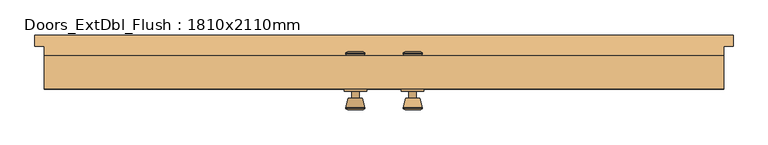
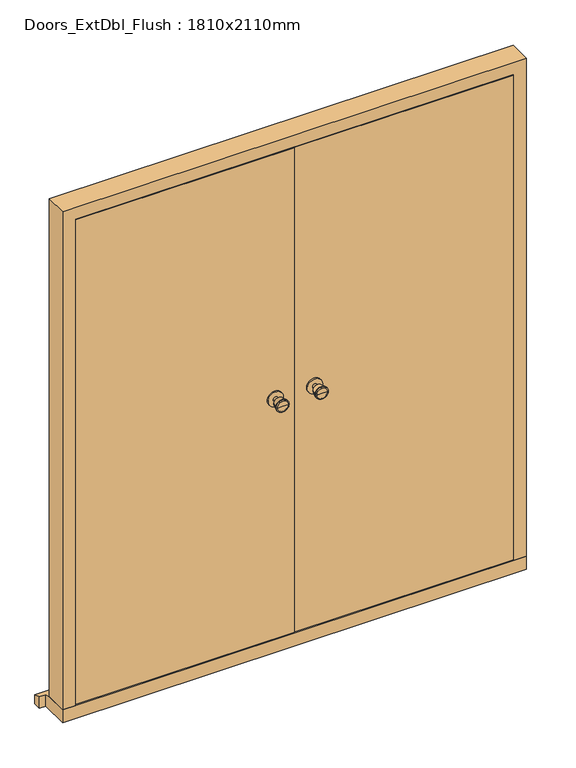
"""IFC4 building model written with IfcOpenShell, lengths in millimetres: door geometry, Doors_ExtDbl_Flush : 1810x2110mm."""

from ifc_helpers import new_model, si_unit, point, frame, frame_2d, origin, place, context, project, spatial, polyline, circle_curve, trimmed, segment, composite_curve, outline, extrude, faceted_brep, source, transform, mapped, element, save
from ifc_brep_helpers import plane_surface, cylinder_surface, revolved_surface, advanced_brep


def doors_extdbl_flush_1810x2110mm_ef948ade(model_context):
    return source(origin(), model_context, "Body", "SolidModel", [
        advanced_brep(
        [(-76.5, -57.5, 1050.0), (-66.5, -57.5, 1050.0), (-86.5, -57.5, 1050.0), (-96.9758676, -106.5, 1050.0), (-56.0241324, -106.5, 1050.0), (-76.5, -106.5, 1050.0), (-101.5, -104.6721319, 1050.0), (-51.5, -104.6721319, 1050.0), (-101.5, -101.2084537, 1050.0), (-51.5, -101.2084537, 1050.0), (-95.136236, -76.5, 1050.0), (-57.863764, -76.5, 1050.0), (-86.5, -76.5, 1050.0), (-66.5, -76.5, 1050.0)],
        [
            (0, 1),
            (1, 2, circle_curve(frame((-76.5, -57.5, 1050.0), z_axis=(0.0, 1.0, 0.0), x_axis=(1.0, 0.0, 0.0)), 10.0)),
            (2, 0),
            (2, 1, circle_curve(frame((-76.5, -57.5, 1050.0), z_axis=(0.0, 1.0, 0.0), x_axis=(1.0, 0.0, 0.0)), 10.0)),
            (3, 4, circle_curve(frame((-76.5, -106.5, 1050.0), z_axis=(0.0, -1.0, 0.0), x_axis=(1.0, 0.0, 0.0)), 20.4758676)),
            (4, 5),
            (5, 3),
            (4, 3, circle_curve(frame((-76.5, -106.5, 1050.0), z_axis=(0.0, -1.0, 0.0), x_axis=(1.0, 0.0, 0.0)), 20.4758676)),
            (6, 7, circle_curve(frame((-76.5, -104.6721319, 1050.0), z_axis=(0.0, -1.0, 0.0), x_axis=(1.0, 0.0, 0.0)), 25.0)),
            (7, 4),
            (3, 6),
            (7, 6, circle_curve(frame((-76.5, -104.6721319, 1050.0), z_axis=(0.0, -1.0, 0.0), x_axis=(1.0, 0.0, 0.0)), 25.0)),
            (8, 9, circle_curve(frame((-76.5, -101.2084537, 1050.0), z_axis=(0.0, -1.0, 0.0), x_axis=(1.0, 0.0, 0.0)), 25.0)),
            (9, 7),
            (6, 8),
            (9, 8, circle_curve(frame((-76.5, -101.2084537, 1050.0), z_axis=(0.0, -1.0, 0.0), x_axis=(1.0, 0.0, 0.0)), 25.0)),
            (10, 11, circle_curve(frame((-76.5, -76.5, 1050.0), z_axis=(0.0, -1.0, 0.0), x_axis=(1.0, 0.0, 0.0)), 18.636236)),
            (11, 9),
            (8, 10),
            (11, 10, circle_curve(frame((-76.5, -76.5, 1050.0), z_axis=(0.0, -1.0, 0.0), x_axis=(1.0, 0.0, 0.0)), 18.636236)),
            (12, 13, circle_curve(frame((-76.5, -76.5, 1050.0), z_axis=(0.0, -1.0, 0.0), x_axis=(1.0, 0.0, 0.0)), 10.0)),
            (13, 11),
            (10, 12),
            (13, 12, circle_curve(frame((-76.5, -76.5, 1050.0), z_axis=(0.0, -1.0, 0.0), x_axis=(1.0, 0.0, 0.0)), 10.0)),
            (1, 13),
            (12, 2),
        ],
        [
            plane_surface(frame((-76.5, -57.5, 1050.0), z_axis=(0.0, 1.0, 0.0), x_axis=(1.0, 0.0, 0.0))),
            plane_surface(frame((-76.5, -106.5, 1050.0), z_axis=(0.0, -1.0, 0.0), x_axis=(1.0, 0.0, 0.0))),
            revolved_surface(polyline([(-56.0241324, -106.5, 1050.0), (-51.5, -104.6721319, 1050.0)]), (-76.5, -57.5, 1050.0), (0.0, 1.0, 0.0)),
            cylinder_surface(frame((-76.5, -57.5, 1050.0), z_axis=(0.0, 1.0, 0.0), x_axis=(1.0, 0.0, 0.0)), 25.0),
            revolved_surface(polyline([(-51.5, -101.2084537, 1050.0), (-57.863764, -76.5, 1050.0)]), (-76.5, -57.5, 1050.0), (0.0, 1.0, 0.0)),
            plane_surface(frame((-76.5, -76.5, 1050.0), z_axis=(0.0, 1.0, 0.0), x_axis=(1.0, 0.0, 0.0))),
            cylinder_surface(frame((-76.5, -57.5, 1050.0), z_axis=(0.0, 1.0, 0.0), x_axis=(1.0, 0.0, 0.0)), 10.0),
        ],
        [
            (0, [[1, 2, 3]]),
            (0, [[-3, 4, -1]]),
            (1, [[5, 6, 7]]),
            (1, [[8, -7, -6]]),
            (2, [[9, 10, -5, 11]]),
            (2, [[12, -11, -8, -10]]),
            (3, [[13, 14, -9, 15]]),
            (3, [[16, -15, -12, -14]]),
            (4, [[17, 18, -13, 19]]),
            (4, [[20, -19, -16, -18]]),
            (5, [[21, 22, -17, 23]]),
            (5, [[24, -23, -20, -22]]),
            (6, [[-2, 25, -21, 26]]),
            (6, [[-4, -26, -24, -25]]),
        ],
    ),
        extrude(outline(composite_curve([segment(trimmed(circle_curve(frame_2d((1050.0, -76.5)), 30.0), [point((1050.0, -46.5))], [point((1050.0, -106.5))], False, "CARTESIAN"), True, "CONTINUOUS"), segment(trimmed(circle_curve(frame_2d((1050.0, -76.5)), 30.0), [point((1050.0, -106.5))], [point((1050.0, -46.5))], False, "CARTESIAN"), True, "CONTINUOUS")], self_intersect=False)), frame((0.0, -57.5, 0.0), z_axis=(0.0, 1.0, 0.0), x_axis=(0.0, 0.0, 1.0)), (0.0, 0.0, 1.0), 6.0),
        advanced_brep(
        [(-76.5, -1.5, 1050.0), (-86.5, -1.5, 1050.0), (-66.5, -1.5, 1050.0), (-96.9758676, 47.5, 1050.0), (-76.5, 47.5, 1050.0), (-56.0241324, 47.5, 1050.0), (-101.5, 45.6721319, 1050.0), (-51.5, 45.6721319, 1050.0), (-101.5, 42.2084537, 1050.0), (-51.5, 42.2084537, 1050.0), (-95.136236, 17.5, 1050.0), (-57.863764, 17.5, 1050.0), (-86.5, 17.5, 1050.0), (-66.5, 17.5, 1050.0)],
        [
            (0, 1),
            (1, 2, circle_curve(frame((-76.5, -1.5, 1050.0), z_axis=(0.0, -1.0, 0.0), x_axis=(1.0, 0.0, 0.0)), 10.0)),
            (2, 0),
            (2, 1, circle_curve(frame((-76.5, -1.5, 1050.0), z_axis=(0.0, -1.0, 0.0), x_axis=(1.0, 0.0, 0.0)), 10.0)),
            (3, 4),
            (4, 5),
            (5, 3, circle_curve(frame((-76.5, 47.5, 1050.0), z_axis=(0.0, 1.0, 0.0), x_axis=(1.0, 0.0, 0.0)), 20.4758676)),
            (3, 5, circle_curve(frame((-76.5, 47.5, 1050.0), z_axis=(0.0, 1.0, 0.0), x_axis=(1.0, 0.0, 0.0)), 20.4758676)),
            (6, 3),
            (5, 7),
            (7, 6, circle_curve(frame((-76.5, 45.6721319, 1050.0), z_axis=(0.0, 1.0, 0.0), x_axis=(1.0, 0.0, 0.0)), 25.0)),
            (6, 7, circle_curve(frame((-76.5, 45.6721319, 1050.0), z_axis=(0.0, 1.0, 0.0), x_axis=(1.0, 0.0, 0.0)), 25.0)),
            (8, 6),
            (7, 9),
            (9, 8, circle_curve(frame((-76.5, 42.2084537, 1050.0), z_axis=(0.0, 1.0, 0.0), x_axis=(1.0, 0.0, 0.0)), 25.0)),
            (8, 9, circle_curve(frame((-76.5, 42.2084537, 1050.0), z_axis=(0.0, 1.0, 0.0), x_axis=(1.0, 0.0, 0.0)), 25.0)),
            (10, 8),
            (9, 11),
            (11, 10, circle_curve(frame((-76.5, 17.5, 1050.0), z_axis=(0.0, 1.0, 0.0), x_axis=(1.0, 0.0, 0.0)), 18.636236)),
            (10, 11, circle_curve(frame((-76.5, 17.5, 1050.0), z_axis=(0.0, 1.0, 0.0), x_axis=(1.0, 0.0, 0.0)), 18.636236)),
            (12, 10),
            (11, 13),
            (13, 12, circle_curve(frame((-76.5, 17.5, 1050.0), z_axis=(0.0, 1.0, 0.0), x_axis=(1.0, 0.0, 0.0)), 10.0)),
            (12, 13, circle_curve(frame((-76.5, 17.5, 1050.0), z_axis=(0.0, 1.0, 0.0), x_axis=(1.0, 0.0, 0.0)), 10.0)),
            (1, 12),
            (13, 2),
        ],
        [
            plane_surface(frame((-76.5, -1.5, 1050.0), z_axis=(0.0, -1.0, 0.0), x_axis=(1.0, 0.0, 0.0))),
            plane_surface(frame((-76.5, 47.5, 1050.0), z_axis=(0.0, 1.0, 0.0), x_axis=(1.0, 0.0, 0.0))),
            revolved_surface(polyline([(-56.0241324, 47.5, 1050.0), (-51.5, 45.6721319, 1050.0)]), (-76.5, -1.5, 1050.0), (0.0, -1.0, 0.0)),
            cylinder_surface(frame((-76.5, -1.5, 1050.0), z_axis=(0.0, -1.0, 0.0), x_axis=(1.0, 0.0, 0.0)), 25.0),
            revolved_surface(polyline([(-51.5, 42.2084537, 1050.0), (-57.863764, 17.5, 1050.0)]), (-76.5, -1.5, 1050.0), (0.0, -1.0, 0.0)),
            plane_surface(frame((-76.5, 17.5, 1050.0), z_axis=(0.0, -1.0, 0.0), x_axis=(1.0, 0.0, 0.0))),
            cylinder_surface(frame((-76.5, -1.5, 1050.0), z_axis=(0.0, -1.0, 0.0), x_axis=(1.0, 0.0, 0.0)), 10.0),
        ],
        [
            (0, [[1, 2, 3]]),
            (0, [[-3, 4, -1]]),
            (1, [[5, 6, 7]]),
            (1, [[-6, -5, 8]]),
            (2, [[9, -7, 10, 11]]),
            (2, [[-10, -8, -9, 12]]),
            (3, [[13, -11, 14, 15]]),
            (3, [[-14, -12, -13, 16]]),
            (4, [[17, -15, 18, 19]]),
            (4, [[-18, -16, -17, 20]]),
            (5, [[21, -19, 22, 23]]),
            (5, [[-22, -20, -21, 24]]),
            (6, [[25, -23, 26, -2]]),
            (6, [[-26, -24, -25, -4]]),
        ],
    ),
        extrude(outline(composite_curve([segment(trimmed(circle_curve(frame_2d((1050.0, -76.5)), 30.0), [point((1050.0, -46.5))], [point((1050.0, -106.5))], False, "CARTESIAN"), True, "CONTINUOUS"), segment(trimmed(circle_curve(frame_2d((1050.0, -76.5)), 30.0), [point((1050.0, -106.5))], [point((1050.0, -46.5))], False, "CARTESIAN"), True, "CONTINUOUS")], self_intersect=False)), frame((0.0, -7.5, 0.0), z_axis=(0.0, 1.0, 0.0), x_axis=(0.0, 0.0, 1.0)), (0.0, 0.0, 1.0), 6.0),
        advanced_brep(
        [(76.5, -57.5, 1050.0), (86.5, -57.5, 1050.0), (66.5, -57.5, 1050.0), (96.9758676, -106.5, 1050.0), (76.5, -106.5, 1050.0), (56.0241324, -106.5, 1050.0), (101.5, -104.6721319, 1050.0), (51.5, -104.6721319, 1050.0), (101.5, -101.2084537, 1050.0), (51.5, -101.2084537, 1050.0), (95.136236, -76.5, 1050.0), (57.863764, -76.5, 1050.0), (86.5, -76.5, 1050.0), (66.5, -76.5, 1050.0)],
        [
            (0, 1),
            (1, 2, circle_curve(frame((76.5, -57.5, 1050.0), z_axis=(0.0, 1.0, 0.0), x_axis=(-1.0, 0.0, 0.0)), 10.0)),
            (2, 0),
            (2, 1, circle_curve(frame((76.5, -57.5, 1050.0), z_axis=(0.0, 1.0, 0.0), x_axis=(-1.0, 0.0, 0.0)), 10.0)),
            (3, 4),
            (4, 5),
            (5, 3, circle_curve(frame((76.5, -106.5, 1050.0), z_axis=(0.0, -1.0, 0.0), x_axis=(-1.0, 0.0, 0.0)), 20.4758676)),
            (3, 5, circle_curve(frame((76.5, -106.5, 1050.0), z_axis=(0.0, -1.0, 0.0), x_axis=(-1.0, 0.0, 0.0)), 20.4758676)),
            (6, 3),
            (5, 7),
            (7, 6, circle_curve(frame((76.5, -104.6721319, 1050.0), z_axis=(0.0, -1.0, 0.0), x_axis=(-1.0, 0.0, 0.0)), 25.0)),
            (6, 7, circle_curve(frame((76.5, -104.6721319, 1050.0), z_axis=(0.0, -1.0, 0.0), x_axis=(-1.0, 0.0, 0.0)), 25.0)),
            (8, 6),
            (7, 9),
            (9, 8, circle_curve(frame((76.5, -101.2084537, 1050.0), z_axis=(0.0, -1.0, 0.0), x_axis=(-1.0, 0.0, 0.0)), 25.0)),
            (8, 9, circle_curve(frame((76.5, -101.2084537, 1050.0), z_axis=(0.0, -1.0, 0.0), x_axis=(-1.0, 0.0, 0.0)), 25.0)),
            (10, 8),
            (9, 11),
            (11, 10, circle_curve(frame((76.5, -76.5, 1050.0), z_axis=(0.0, -1.0, 0.0), x_axis=(-1.0, 0.0, 0.0)), 18.636236)),
            (10, 11, circle_curve(frame((76.5, -76.5, 1050.0), z_axis=(0.0, -1.0, 0.0), x_axis=(-1.0, 0.0, 0.0)), 18.636236)),
            (12, 10),
            (11, 13),
            (13, 12, circle_curve(frame((76.5, -76.5, 1050.0), z_axis=(0.0, -1.0, 0.0), x_axis=(-1.0, 0.0, 0.0)), 10.0)),
            (12, 13, circle_curve(frame((76.5, -76.5, 1050.0), z_axis=(0.0, -1.0, 0.0), x_axis=(-1.0, 0.0, 0.0)), 10.0)),
            (1, 12),
            (13, 2),
        ],
        [
            plane_surface(frame((76.5, -57.5, 1050.0), z_axis=(0.0, 1.0, 0.0), x_axis=(-1.0, 0.0, 0.0))),
            plane_surface(frame((76.5, -106.5, 1050.0), z_axis=(0.0, -1.0, 0.0), x_axis=(-1.0, 0.0, 0.0))),
            revolved_surface(polyline([(56.0241324, -106.5, 1050.0), (51.5, -104.6721319, 1050.0)]), (76.5, -57.5, 1050.0), (0.0, 1.0, 0.0)),
            cylinder_surface(frame((76.5, -57.5, 1050.0), z_axis=(0.0, 1.0, 0.0), x_axis=(-1.0, 0.0, 0.0)), 25.0),
            revolved_surface(polyline([(51.5, -101.2084537, 1050.0), (57.863764, -76.5, 1050.0)]), (76.5, -57.5, 1050.0), (0.0, 1.0, 0.0)),
            plane_surface(frame((76.5, -76.5, 1050.0), z_axis=(0.0, 1.0, 0.0), x_axis=(-1.0, 0.0, 0.0))),
            cylinder_surface(frame((76.5, -57.5, 1050.0), z_axis=(0.0, 1.0, 0.0), x_axis=(-1.0, 0.0, 0.0)), 10.0),
        ],
        [
            (0, [[1, 2, 3]]),
            (0, [[-3, 4, -1]]),
            (1, [[5, 6, 7]]),
            (1, [[-6, -5, 8]]),
            (2, [[9, -7, 10, 11]]),
            (2, [[-10, -8, -9, 12]]),
            (3, [[13, -11, 14, 15]]),
            (3, [[-14, -12, -13, 16]]),
            (4, [[17, -15, 18, 19]]),
            (4, [[-18, -16, -17, 20]]),
            (5, [[21, -19, 22, 23]]),
            (5, [[-22, -20, -21, 24]]),
            (6, [[25, -23, 26, -2]]),
            (6, [[-26, -24, -25, -4]]),
        ],
    ),
        extrude(outline(composite_curve([segment(trimmed(circle_curve(frame_2d((1050.0, 76.5)), 30.0), [point((1050.0, 46.5))], [point((1050.0, 106.5))], False, "CARTESIAN"), True, "CONTINUOUS"), segment(trimmed(circle_curve(frame_2d((1050.0, 76.5)), 30.0), [point((1050.0, 106.5))], [point((1050.0, 46.5))], False, "CARTESIAN"), True, "CONTINUOUS")], self_intersect=False)), frame((0.0, -57.5, 0.0), z_axis=(0.0, 1.0, 0.0), x_axis=(0.0, 0.0, 1.0)), (0.0, 0.0, 1.0), 6.0),
        advanced_brep(
        [(76.5, -1.5, 1050.0), (66.5, -1.5, 1050.0), (86.5, -1.5, 1050.0), (96.9758676, 47.5, 1050.0), (56.0241324, 47.5, 1050.0), (76.5, 47.5, 1050.0), (101.5, 45.6721319, 1050.0), (51.5, 45.6721319, 1050.0), (101.5, 42.2084537, 1050.0), (51.5, 42.2084537, 1050.0), (95.136236, 17.5, 1050.0), (57.863764, 17.5, 1050.0), (86.5, 17.5, 1050.0), (66.5, 17.5, 1050.0)],
        [
            (0, 1),
            (1, 2, circle_curve(frame((76.5, -1.5, 1050.0), z_axis=(0.0, -1.0, 0.0), x_axis=(-1.0, 0.0, 0.0)), 10.0)),
            (2, 0),
            (2, 1, circle_curve(frame((76.5, -1.5, 1050.0), z_axis=(0.0, -1.0, 0.0), x_axis=(-1.0, 0.0, 0.0)), 10.0)),
            (3, 4, circle_curve(frame((76.5, 47.5, 1050.0), z_axis=(0.0, 1.0, 0.0), x_axis=(-1.0, 0.0, 0.0)), 20.4758676)),
            (4, 5),
            (5, 3),
            (4, 3, circle_curve(frame((76.5, 47.5, 1050.0), z_axis=(0.0, 1.0, 0.0), x_axis=(-1.0, 0.0, 0.0)), 20.4758676)),
            (6, 7, circle_curve(frame((76.5, 45.6721319, 1050.0), z_axis=(0.0, 1.0, 0.0), x_axis=(-1.0, 0.0, 0.0)), 25.0)),
            (7, 4),
            (3, 6),
            (7, 6, circle_curve(frame((76.5, 45.6721319, 1050.0), z_axis=(0.0, 1.0, 0.0), x_axis=(-1.0, 0.0, 0.0)), 25.0)),
            (8, 9, circle_curve(frame((76.5, 42.2084537, 1050.0), z_axis=(0.0, 1.0, 0.0), x_axis=(-1.0, 0.0, 0.0)), 25.0)),
            (9, 7),
            (6, 8),
            (9, 8, circle_curve(frame((76.5, 42.2084537, 1050.0), z_axis=(0.0, 1.0, 0.0), x_axis=(-1.0, 0.0, 0.0)), 25.0)),
            (10, 11, circle_curve(frame((76.5, 17.5, 1050.0), z_axis=(0.0, 1.0, 0.0), x_axis=(-1.0, 0.0, 0.0)), 18.636236)),
            (11, 9),
            (8, 10),
            (11, 10, circle_curve(frame((76.5, 17.5, 1050.0), z_axis=(0.0, 1.0, 0.0), x_axis=(-1.0, 0.0, 0.0)), 18.636236)),
            (12, 13, circle_curve(frame((76.5, 17.5, 1050.0), z_axis=(0.0, 1.0, 0.0), x_axis=(-1.0, 0.0, 0.0)), 10.0)),
            (13, 11),
            (10, 12),
            (13, 12, circle_curve(frame((76.5, 17.5, 1050.0), z_axis=(0.0, 1.0, 0.0), x_axis=(-1.0, 0.0, 0.0)), 10.0)),
            (1, 13),
            (12, 2),
        ],
        [
            plane_surface(frame((76.5, -1.5, 1050.0), z_axis=(0.0, -1.0, 0.0), x_axis=(-1.0, 0.0, 0.0))),
            plane_surface(frame((76.5, 47.5, 1050.0), z_axis=(0.0, 1.0, 0.0), x_axis=(-1.0, 0.0, 0.0))),
            revolved_surface(polyline([(56.0241324, 47.5, 1050.0), (51.5, 45.6721319, 1050.0)]), (76.5, -1.5, 1050.0), (0.0, -1.0, 0.0)),
            cylinder_surface(frame((76.5, -1.5, 1050.0), z_axis=(0.0, -1.0, 0.0), x_axis=(-1.0, 0.0, 0.0)), 25.0),
            revolved_surface(polyline([(51.5, 42.2084537, 1050.0), (57.863764, 17.5, 1050.0)]), (76.5, -1.5, 1050.0), (0.0, -1.0, 0.0)),
            plane_surface(frame((76.5, 17.5, 1050.0), z_axis=(0.0, -1.0, 0.0), x_axis=(-1.0, 0.0, 0.0))),
            cylinder_surface(frame((76.5, -1.5, 1050.0), z_axis=(0.0, -1.0, 0.0), x_axis=(-1.0, 0.0, 0.0)), 10.0),
        ],
        [
            (0, [[1, 2, 3]]),
            (0, [[-3, 4, -1]]),
            (1, [[5, 6, 7]]),
            (1, [[8, -7, -6]]),
            (2, [[9, 10, -5, 11]]),
            (2, [[12, -11, -8, -10]]),
            (3, [[13, 14, -9, 15]]),
            (3, [[16, -15, -12, -14]]),
            (4, [[17, 18, -13, 19]]),
            (4, [[20, -19, -16, -18]]),
            (5, [[21, 22, -17, 23]]),
            (5, [[24, -23, -20, -22]]),
            (6, [[-2, 25, -21, 26]]),
            (6, [[-4, -26, -24, -25]]),
        ],
    ),
        extrude(outline(composite_curve([segment(trimmed(circle_curve(frame_2d((1050.0, 76.5)), 30.0), [point((1050.0, 46.5))], [point((1050.0, 106.5))], False, "CARTESIAN"), True, "CONTINUOUS"), segment(trimmed(circle_curve(frame_2d((1050.0, 76.5)), 30.0), [point((1050.0, 106.5))], [point((1050.0, 46.5))], False, "CARTESIAN"), True, "CONTINUOUS")], self_intersect=False)), frame((0.0, -7.5, 0.0), z_axis=(0.0, 1.0, 0.0), x_axis=(0.0, 0.0, 1.0)), (0.0, 0.0, 1.0), 6.0),
        faceted_brep([(834.5, 37.5, 54.5), (905.0, 37.5, 54.5), (905.0, -51.5, 54.5), (856.5, -51.5, 54.5), (856.5, -4.5, 54.5), (834.5, -4.5, 54.5), (834.5, 37.5, 2039.5), (-834.5, 37.5, 2039.5), (-834.5, 37.5, 54.5), (-905.0, 37.5, 54.5), (-905.0, 37.5, 2110.0), (905.0, 37.5, 2110.0), (905.0, -51.5, 2110.0), (-905.0, -51.5, 2110.0), (-905.0, -51.5, 54.5), (-856.5, -51.5, 54.5), (-856.5, -51.5, 2061.5), (856.5, -51.5, 2061.5), (856.5, -4.5, 2061.5), (-856.5, -4.5, 2061.5), (-856.5, -4.5, 54.5), (-834.5, -4.5, 54.5), (-834.5, -4.5, 2039.5), (834.5, -4.5, 2039.5)], [[[0, 1, 2, 3, 4, 5]], [[1, 0, 6, 7, 8, 9, 10, 11]], [[2, 1, 11, 12]], [[3, 2, 12, 13, 14, 15, 16, 17]], [[4, 3, 17, 18]], [[5, 4, 18, 19, 20, 21, 22, 23]], [[0, 5, 23, 6]], [[12, 11, 10, 13]], [[18, 17, 16, 19]], [[6, 23, 22, 7]], [[8, 21, 20, 15, 14, 9]], [[13, 10, 9, 14]], [[19, 16, 15, 20]], [[7, 22, 21, 8]]]),
        faceted_brep([(930.0, 92.5, 0.0), (930.0, 92.5, 38.5947221), (930.0, 62.5, 47.2703282), (930.0, 62.5, 0.0), (-930.0, 92.5, 38.5947221), (-930.0, 92.5, 0.0), (-930.0, 62.5, 0.0), (-930.0, 62.5, 47.2703282), (905.0, 62.5, 0.0), (905.0, -51.5, 0.0), (-905.0, -51.5, 0.0), (-905.0, 62.5, 0.0), (-905.0, 62.5, 47.2703282), (-905.0, 37.5, 54.5), (905.0, 37.5, 54.5), (905.0, 62.5, 47.2703282), (-905.0, -51.5, 54.5), (905.0, -51.5, 54.5)], [[[0, 1, 2, 3]], [[4, 5, 6, 7]], [[5, 0, 3, 8, 9, 10, 11, 6]], [[1, 0, 5, 4]], [[1, 4, 7, 12, 13, 14, 15, 2]], [[13, 16, 17, 14]], [[16, 10, 9, 17]], [[12, 11, 10, 16, 13]], [[11, 12, 7, 6]], [[8, 15, 14, 17, 9]], [[15, 8, 3, 2]]]),
        extrude(outline(polyline([(853.5, -51.5), (1.5, -51.5), (1.5, -7.5), (853.5, -7.5), (853.5, -51.5)])), frame((0.0, 0.0, 58.5), z_axis=(0.0, 0.0, 1.0), x_axis=(1.0, 0.0, 0.0)), (0.0, 0.0, 1.0), 2000.0),
        extrude(outline(polyline([(-1.5, -51.5), (-853.5, -51.5), (-853.5, -7.5), (-1.5, -7.5), (-1.5, -51.5)])), frame((0.0, 0.0, 58.5), z_axis=(0.0, 0.0, 1.0), x_axis=(1.0, 0.0, 0.0)), (0.0, 0.0, 1.0), 2000.0),
    ])


if __name__ == "__main__":
    model = new_model("IFC4")
    model_context = context("Model", 3, world=origin())
    ifc_project = project(units=[si_unit("LENGTHUNIT", "METRE", prefix="MILLI")], contexts=[model_context])
    site = spatial("IfcSite", under=ifc_project)
    building = spatial("IfcBuilding", under=site)
    placement = place(None, origin())
    doors_extdbl_flush_1810x2110mm_shape = doors_extdbl_flush_1810x2110mm_ef948ade(model_context)
    element("IfcDoor", 1, ObjectType="Doors_ExtDbl_Flush : 1810x2110mm", at=placement, inside=building, context=model_context, shape_type="MappedRepresentation", body=[
        mapped(doors_extdbl_flush_1810x2110mm_shape, transform((0.0, 0.0, 0.0), x_axis=(1.0, 0.0, 0.0), y_axis=(0.0, 1.0, 0.0), z_axis=(0.0, 0.0, 1.0))),
    ])
    save(model, "model.ifc")

# Revit data of these elements
# Type "Doors_ExtDbl_Flush : 1810x2110mm"
#   Type Mark = "44"
#   Type Comments = "External Double"
#   Operation = "DoubleDoorSingleSwing"
#   Keynote = "L20"
#   Analytic Construction = "Metal"
#   Wrap Layers (Ext) from Ext = 102.5 mm
#   Wrap Layers (Int) from Ext = 177.5 mm
#   Thickness = 44 mm
#   Rough Width = 1810 mm
#   Rough Height = 2110 mm
#   O/A Frame Width = 64 mm
#   Heat Transfer Coefficient (U) = 3.7021 W/(m²·K)
#   Handle Z Distance = 1050 mm
#   FrameWidth = 42 mm
#   FrameOffset - External = 25 mm
#   FrameDepth = 89 mm
#   Door Panel Width = 852 mm
#   Door Panel Thickness = 44 mm
#   Door Panel Height = 2000 mm
#   Cill Thickness = 54.5 mm
#   Cill Projection = 30 mm
#   Handle X Distance = 75 mm
#   Height = 2110 mm
#   Structural Tolerance = 6.5 mm
#   Tolerance = 3 mm
#   Undercut = 4 mm
#   Width = 1810 mm
#   Cill Extension = 25 mm
#   Cavity Closer Width = 50 mm
#   Cavity Closer Offset from Ext = 102.5 mm
#   Cavity Closer Depth = 85 mm
#   Vis - Ironmongery = yes
#   Vis - Cavity Closers = yes
#   Function = 1
#   Material Door = Door - Panel
#   Material Frame = Door - Frame/Mullion
#   Material Ironmongery = Door - Handle
#   Visual Light Transmittance = 0
#   Thermal Resistance (R) = 0
#   Solar Heat Gain Coefficient = 0
#   Wall Closure = (empty or 0)
# Element 1 (IfcDoor, "Doors_ExtDbl_Flush : 1810x2110mm")
#   Materials on its faces: "Door - Handle", "Door - Frame/Mullion", "Door - Panel"
# Materials
#   "Door - Panel": class "Wood", colour RGB 210 159 95, transparency 0, Keynote = "L20"
#   "Door - Frame/Mullion": class "Wood", colour RGB 212 179 113, transparency 0, Keynote = "L20"
#   "Door - Handle": class "Miscellaneous", colour RGB 0 0 0, transparency 0, Keynote = "P21"
